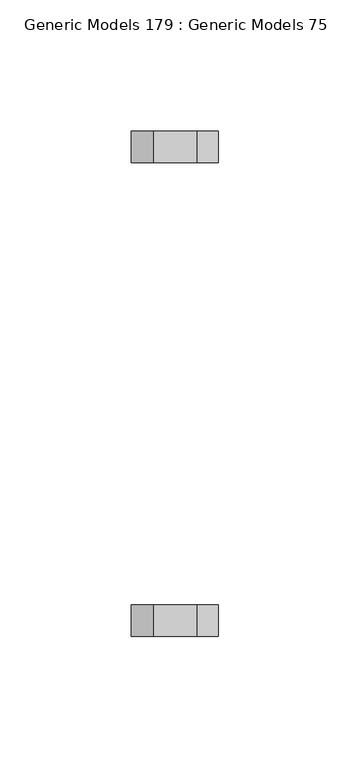
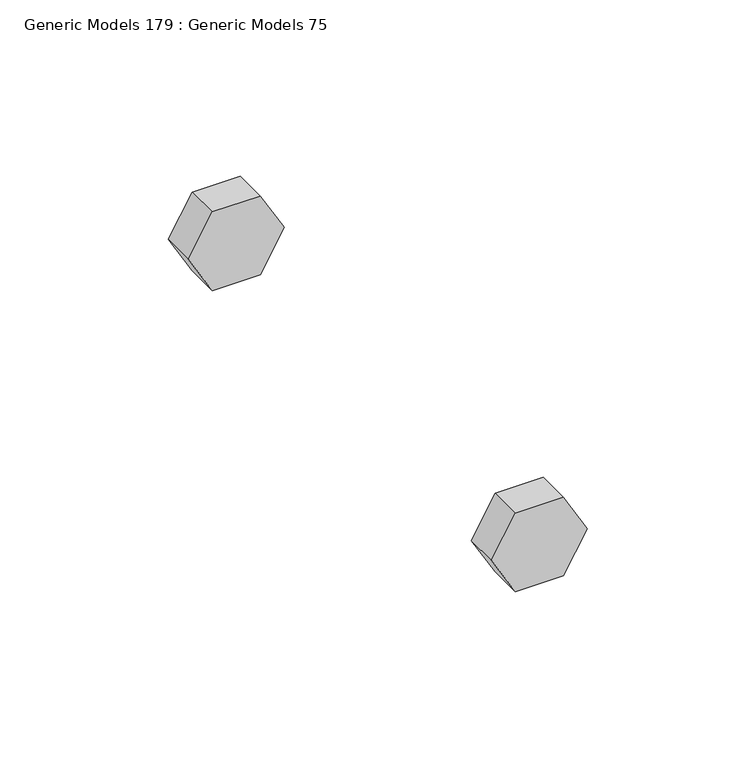
"""IFC4 building model written with IfcOpenShell, lengths in millimetres: proxy geometry, Generic Models 179 : Generic Models 75."""

from ifc_helpers import new_model, si_unit, frame, origin, place, context, project, spatial, polyline, outline, extrude, source, transform, mapped, element, save


def generic_models_179_generic_models_75_1166544c(model_context):
    return source(origin(), model_context, "Body", "SweptSolid", [
        extrude(outline(polyline([(271733.9625, 31979.8726858), (271733.9625, 31996.3704698), (271748.25, 32004.6193618), (271762.5375, 31996.3704698), (271762.5375, 31979.8726858), (271748.25, 31971.6237939), (271733.9625, 31979.8726858)])), frame((0.0, 36311.3770442, 0.0), z_axis=(0.0, 1.0, 0.0), x_axis=(0.0, 0.0, 1.0)), (0.0, 0.0, 1.0), 11.90625),
        extrude(outline(polyline([(271733.9625, 31979.8726858), (271733.9625, 31996.3704698), (271748.25, 32004.6193618), (271762.5375, 31996.3704698), (271762.5375, 31979.8726858), (271748.25, 31971.6237939), (271733.9625, 31979.8726858)])), frame((0.0, 36491.5582942, 0.0), z_axis=(0.0, 1.0, 0.0), x_axis=(0.0, 0.0, 1.0)), (0.0, 0.0, 1.0), 11.90625),
    ])


if __name__ == "__main__":
    model = new_model("IFC4")
    model_context = context("Model", 3, world=origin())
    ifc_project = project(units=[si_unit("LENGTHUNIT", "METRE", prefix="MILLI")], contexts=[model_context])
    site = spatial("IfcSite", under=ifc_project)
    building = spatial("IfcBuilding", under=site)
    placement = place(None, origin())
    generic_models_179_generic_models_75_shape = generic_models_179_generic_models_75_1166544c(model_context)
    element("IfcBuildingElementProxy", 1, Name="Generic Models 179 : Generic Models 75", ObjectType="Generic Models 179 : Generic Models 75", at=placement, inside=building, context=model_context, shape_type="MappedRepresentation", body=[
        mapped(generic_models_179_generic_models_75_shape, transform((0.0, 0.0, 0.0), x_axis=(1.0, 0.0, 0.0), y_axis=(0.0, 1.0, 0.0), z_axis=(0.0, 0.0, 1.0))),
    ])
    save(model, "model.ifc")

# Revit data of these elements
# Element 1 (IfcBuildingElementProxy, "Generic Models 179 : Generic Models 75")
#   Materials on its faces: "3/4\" GALV. THRU BOLTS"
# Materials
#   "3/4\" GALV. THRU BOLTS": class "Generic", colour RGB 105 69 171, transparency 0, Cost = 0
